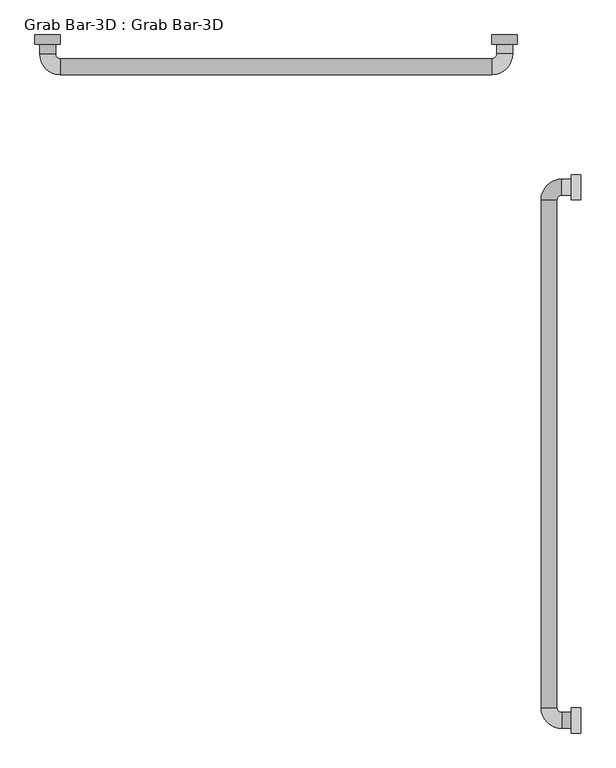
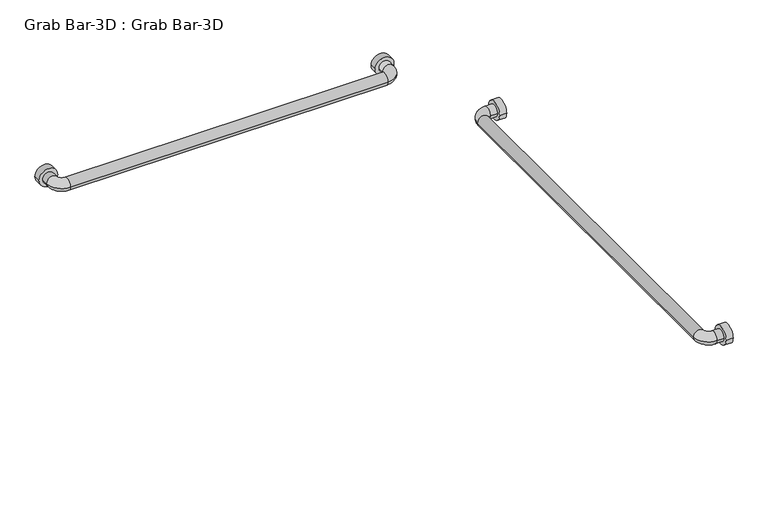
"""IFC4 building model written with IfcOpenShell, lengths in millimetres: proxy geometry, Grab Bar-3D : Grab Bar-3D."""

from ifc_helpers import new_model, si_unit, point, frame, frame_2d, origin, place, context, project, spatial, circle_curve, ellipse_curve, trimmed, segment, composite_curve, outline, extrude, source, transform, mapped, element, save
from ifc_brep_helpers import plane_surface, cylinder_surface, revolved_surface, advanced_brep


def grab_bar_3d_grab_bar_3d_a3ed3e83(model_context):
    return source(origin(), model_context, "Body", "SolidModel", [
        extrude(outline(composite_curve([segment(trimmed(circle_curve(frame_2d((-304.8, 914.4)), 25.4), [point((-279.4, 914.4))], [point((-330.2, 914.4))], False, "CARTESIAN"), True, "CONTINUOUS"), segment(trimmed(circle_curve(frame_2d((-304.8, 914.4)), 25.4), [point((-330.2, 914.4))], [point((-279.4, 914.4))], False, "CARTESIAN"), True, "CONTINUOUS")], self_intersect=False)), frame((-19.05, 0.0, 0.0), z_axis=(1.0, 0.0, 0.0), x_axis=(0.0, 1.0, 0.0)), (0.0, 0.0, 1.0), 19.05),
        extrude(outline(composite_curve([segment(trimmed(circle_curve(frame_2d((-1371.6, 914.4)), 25.4), [point((-1346.2, 914.4))], [point((-1397.0, 914.4))], False, "CARTESIAN"), True, "CONTINUOUS"), segment(trimmed(circle_curve(frame_2d((-1371.6, 914.4)), 25.4), [point((-1397.0, 914.4))], [point((-1346.2, 914.4))], False, "CARTESIAN"), True, "CONTINUOUS")], self_intersect=False)), frame((-19.05, 0.0, 0.0), z_axis=(1.0, 0.0, 0.0), x_axis=(0.0, 1.0, 0.0)), (0.0, 0.0, 1.0), 19.05),
        extrude(outline(composite_curve([segment(trimmed(circle_curve(frame_2d((914.4, -152.4)), 25.4), [point((914.4, -177.8))], [point((914.4, -127.0))], False, "CARTESIAN"), True, "CONTINUOUS"), segment(trimmed(circle_curve(frame_2d((914.4, -152.4)), 25.4), [point((914.4, -127.0))], [point((914.4, -177.8))], False, "CARTESIAN"), True, "CONTINUOUS")], self_intersect=False)), frame((0.0, -19.05, 0.0), z_axis=(0.0, 1.0, 0.0), x_axis=(0.0, 0.0, 1.0)), (0.0, 0.0, 1.0), 19.05),
        extrude(outline(composite_curve([segment(trimmed(circle_curve(frame_2d((914.4, -1066.8)), 25.4), [point((914.4, -1092.2))], [point((914.4, -1041.4))], False, "CARTESIAN"), True, "CONTINUOUS"), segment(trimmed(circle_curve(frame_2d((914.4, -1066.8)), 25.4), [point((914.4, -1041.4))], [point((914.4, -1092.2))], False, "CARTESIAN"), True, "CONTINUOUS")], self_intersect=False)), frame((0.0, -19.05, 0.0), z_axis=(0.0, 1.0, 0.0), x_axis=(0.0, 0.0, 1.0)), (0.0, 0.0, 1.0), 19.05),
        advanced_brep(
        [(-19.05, -320.675, 914.4), (-19.05, -288.925, 914.4), (-38.1, -288.925, 914.4), (-38.1, -320.675, 914.4), (-79.375, -330.2, 914.4), (-47.625, -330.2, 914.4), (-79.375, -1346.2, 914.4), (-47.625, -1346.2, 914.4), (-38.1, -1387.475, 914.4), (-38.1, -1355.725, 914.4), (-19.05, -1355.725, 914.4), (-19.05, -1387.475, 914.4)],
        [
            (0, 1, circle_curve(frame((-19.05, -304.8, 914.4), z_axis=(1.0, 0.0, 0.0), x_axis=(0.0, 1.0, 0.0)), 15.875)),
            (1, 0, circle_curve(frame((-19.05, -304.8, 914.4), z_axis=(1.0, 0.0, 0.0), x_axis=(0.0, 1.0, 0.0)), 15.875)),
            (1, 2),
            (2, 3, circle_curve(frame((-38.1, -304.8, 914.4), z_axis=(1.0, 0.0, 0.0), x_axis=(0.0, 1.0, 0.0)), 15.875)),
            (3, 0),
            (3, 2, circle_curve(frame((-38.1, -304.8, 914.4), z_axis=(1.0, 0.0, 0.0), x_axis=(0.0, 1.0, 0.0)), 15.875)),
            (4, 5, circle_curve(frame((-63.5, -330.2, 914.4), z_axis=(0.0, 1.0, 0.0), x_axis=(-1.0, 0.0, 0.0)), 15.875)),
            (5, 3, circle_curve(frame((-38.1, -330.2, 914.4), z_axis=(0.0, 0.0, -1.0), x_axis=(0.0, 1.0, 0.0)), 9.525)),
            (2, 4, circle_curve(frame((-38.1, -330.2, 914.4), z_axis=(0.0, 0.0, 1.0), x_axis=(0.0, 1.0, 0.0)), 41.275)),
            (5, 4, circle_curve(frame((-63.5, -330.2, 914.4), z_axis=(0.0, 1.0, 0.0), x_axis=(-1.0, 0.0, 0.0)), 15.875)),
            (4, 6),
            (6, 7, circle_curve(frame((-63.5, -1346.2, 914.4), z_axis=(0.0, 1.0, 0.0), x_axis=(-1.0, 0.0, 0.0)), 15.875)),
            (7, 5),
            (7, 6, circle_curve(frame((-63.5, -1346.2, 914.4), z_axis=(0.0, 1.0, 0.0), x_axis=(-1.0, 0.0, 0.0)), 15.875)),
            (8, 9, circle_curve(frame((-38.1, -1371.6, 914.4), z_axis=(-1.0, 0.0, 0.0), x_axis=(0.0, -1.0, 0.0)), 15.875)),
            (9, 7, circle_curve(frame((-38.1, -1346.2, 914.4), z_axis=(0.0, 0.0, -1.0), x_axis=(-1.0, 0.0, 0.0)), 9.525)),
            (6, 8, circle_curve(frame((-38.1, -1346.2, 914.4), z_axis=(0.0, 0.0, 1.0), x_axis=(-1.0, 0.0, 0.0)), 41.275)),
            (9, 8, circle_curve(frame((-38.1, -1371.6, 914.4), z_axis=(-1.0, 0.0, 0.0), x_axis=(0.0, -1.0, 0.0)), 15.875)),
            (10, 11, circle_curve(frame((-19.05, -1371.6, 914.4), z_axis=(1.0, 0.0, 0.0), x_axis=(0.0, -1.0, 0.0)), 15.875)),
            (11, 10, circle_curve(frame((-19.05, -1371.6, 914.4), z_axis=(1.0, 0.0, 0.0), x_axis=(0.0, -1.0, 0.0)), 15.875)),
            (8, 11),
            (10, 9),
        ],
        [
            plane_surface(frame((-19.05, -304.8, -930.275), z_axis=(1.0, 0.0, 0.0), x_axis=(0.0, 1.0, 0.0))),
            cylinder_surface(frame((-19.05, -304.8, 914.4), z_axis=(1.0, 0.0, 0.0), x_axis=(0.0, 1.0, 0.0)), 15.875),
            revolved_surface(trimmed(ellipse_curve(frame((-38.1, -304.8, 914.4), z_axis=(-1.0, 0.0, 0.0), x_axis=(0.0, 1.0, 0.0)), 15.875, 15.875), [point((-38.1, -320.675, 914.4))], [point((-38.1, -288.925, 914.4))], True, "CARTESIAN"), (-38.1, -330.2, 0.0), (0.0, 0.0, -1.0)),
            revolved_surface(trimmed(ellipse_curve(frame((-38.1, -304.8, 914.4), z_axis=(-1.0, 0.0, 0.0), x_axis=(0.0, 1.0, 0.0)), 15.875, 15.875), [point((-38.1, -288.925, 914.4))], [point((-38.1, -320.675, 914.4))], True, "CARTESIAN"), (-38.1, -330.2, 0.0), (0.0, 0.0, -1.0)),
            cylinder_surface(frame((-63.5, -330.2, 914.4), z_axis=(0.0, 1.0, 0.0), x_axis=(-1.0, 0.0, 0.0)), 15.875),
            revolved_surface(trimmed(ellipse_curve(frame((-63.5, -1346.2, 914.4), z_axis=(0.0, -1.0, 0.0), x_axis=(-1.0, 0.0, 0.0)), 15.875, 15.875), [point((-47.625, -1346.2, 914.4))], [point((-79.375, -1346.2, 914.4))], True, "CARTESIAN"), (-38.1, -1346.2, 0.0), (0.0, 0.0, -1.0)),
            revolved_surface(trimmed(ellipse_curve(frame((-63.5, -1346.2, 914.4), z_axis=(0.0, -1.0, 0.0), x_axis=(-1.0, 0.0, 0.0)), 15.875, 15.875), [point((-79.375, -1346.2, 914.4))], [point((-47.625, -1346.2, 914.4))], True, "CARTESIAN"), (-38.1, -1346.2, 0.0), (0.0, 0.0, -1.0)),
            plane_surface(frame((-19.05, -1371.6, -930.275), z_axis=(1.0, 0.0, 0.0), x_axis=(0.0, -1.0, 0.0))),
            cylinder_surface(frame((-38.1, -1371.6, 914.4), z_axis=(-1.0, 0.0, 0.0), x_axis=(0.0, -1.0, 0.0)), 15.875),
        ],
        [
            (0, [[1, 2]]),
            (1, [[3, 4, 5, -2]]),
            (1, [[-5, 6, -3, -1]]),
            (2, [[7, 8, -4, 9]]),
            (3, [[10, -9, -6, -8]]),
            (4, [[11, 12, 13, -7]]),
            (4, [[-13, 14, -11, -10]]),
            (5, [[15, 16, -12, 17]]),
            (6, [[18, -17, -14, -16]]),
            (7, [[19, 20]]),
            (8, [[21, -19, 22, -15]]),
            (8, [[-22, -20, -21, -18]]),
        ],
    ),
        advanced_brep(
        [(-1050.925, -19.05, 914.4), (-1082.675, -19.05, 914.4), (-1082.675, -38.1, 914.4), (-1050.925, -38.1, 914.4), (-1041.4, -79.375, 914.4), (-1041.4, -47.625, 914.4), (-177.8, -79.375, 914.4), (-177.8, -47.625, 914.4), (-136.525, -38.1, 914.4), (-168.275, -38.1, 914.4), (-168.275, -19.05, 914.4), (-136.525, -19.05, 914.4)],
        [
            (0, 1, circle_curve(frame((-1066.8, -19.05, 914.4), z_axis=(0.0, 1.0, 0.0), x_axis=(-1.0, 0.0, 0.0)), 15.875)),
            (1, 0, circle_curve(frame((-1066.8, -19.05, 914.4), z_axis=(0.0, 1.0, 0.0), x_axis=(-1.0, 0.0, 0.0)), 15.875)),
            (1, 2),
            (2, 3, circle_curve(frame((-1066.8, -38.1, 914.4), z_axis=(0.0, 1.0, 0.0), x_axis=(-1.0, 0.0, 0.0)), 15.875)),
            (3, 0),
            (3, 2, circle_curve(frame((-1066.8, -38.1, 914.4), z_axis=(0.0, 1.0, 0.0), x_axis=(-1.0, 0.0, 0.0)), 15.875)),
            (4, 5, circle_curve(frame((-1041.4, -63.5, 914.4), z_axis=(-1.0, 0.0, 0.0), x_axis=(0.0, -1.0, 0.0)), 15.875)),
            (5, 3, circle_curve(frame((-1041.4, -38.1, 914.4), z_axis=(0.0, 0.0, -1.0), x_axis=(-1.0, 0.0, 0.0)), 9.525)),
            (2, 4, circle_curve(frame((-1041.4, -38.1, 914.4), z_axis=(0.0, 0.0, 1.0), x_axis=(-1.0, 0.0, 0.0)), 41.275)),
            (5, 4, circle_curve(frame((-1041.4, -63.5, 914.4), z_axis=(-1.0, 0.0, 0.0), x_axis=(0.0, -1.0, 0.0)), 15.875)),
            (4, 6),
            (6, 7, circle_curve(frame((-177.8, -63.5, 914.4), z_axis=(-1.0, 0.0, 0.0), x_axis=(0.0, -1.0, 0.0)), 15.875)),
            (7, 5),
            (7, 6, circle_curve(frame((-177.8, -63.5, 914.4), z_axis=(-1.0, 0.0, 0.0), x_axis=(0.0, -1.0, 0.0)), 15.875)),
            (8, 9, circle_curve(frame((-152.4, -38.1, 914.4), z_axis=(0.0, -1.0, 0.0), x_axis=(1.0, 0.0, 0.0)), 15.875)),
            (9, 7, circle_curve(frame((-177.8, -38.1, 914.4), z_axis=(0.0, 0.0, -1.0), x_axis=(0.0, -1.0, 0.0)), 9.525)),
            (6, 8, circle_curve(frame((-177.8, -38.1, 914.4), z_axis=(0.0, 0.0, 1.0), x_axis=(0.0, -1.0, 0.0)), 41.275)),
            (9, 8, circle_curve(frame((-152.4, -38.1, 914.4), z_axis=(0.0, -1.0, 0.0), x_axis=(1.0, 0.0, 0.0)), 15.875)),
            (10, 11, circle_curve(frame((-152.4, -19.05, 914.4), z_axis=(0.0, 1.0, 0.0), x_axis=(1.0, 0.0, 0.0)), 15.875)),
            (11, 10, circle_curve(frame((-152.4, -19.05, 914.4), z_axis=(0.0, 1.0, 0.0), x_axis=(1.0, 0.0, 0.0)), 15.875)),
            (8, 11),
            (10, 9),
        ],
        [
            plane_surface(frame((-1997.075, -19.05, 0.0), z_axis=(0.0, 1.0, 0.0), x_axis=(0.0, 0.0, 1.0))),
            cylinder_surface(frame((-1066.8, -19.05, 914.4), z_axis=(0.0, 1.0, 0.0), x_axis=(-1.0, 0.0, 0.0)), 15.875),
            revolved_surface(trimmed(ellipse_curve(frame((-1066.8, -38.1, 914.4), z_axis=(0.0, -1.0, 0.0), x_axis=(-1.0, 0.0, 0.0)), 15.875, 15.875), [point((-1050.925, -38.1, 914.4))], [point((-1082.675, -38.1, 914.4))], True, "CARTESIAN"), (-1041.4, -38.1, 0.0), (0.0, 0.0, -1.0)),
            revolved_surface(trimmed(ellipse_curve(frame((-1066.8, -38.1, 914.4), z_axis=(0.0, -1.0, 0.0), x_axis=(-1.0, 0.0, 0.0)), 15.875, 15.875), [point((-1082.675, -38.1, 914.4))], [point((-1050.925, -38.1, 914.4))], True, "CARTESIAN"), (-1041.4, -38.1, 0.0), (0.0, 0.0, -1.0)),
            cylinder_surface(frame((-1041.4, -63.5, 914.4), z_axis=(-1.0, 0.0, 0.0), x_axis=(0.0, -1.0, 0.0)), 15.875),
            revolved_surface(trimmed(ellipse_curve(frame((-177.8, -63.5, 914.4), z_axis=(1.0, 0.0, 0.0), x_axis=(0.0, -1.0, 0.0)), 15.875, 15.875), [point((-177.8, -47.625, 914.4))], [point((-177.8, -79.375, 914.4))], True, "CARTESIAN"), (-177.8, -38.1, 0.0), (0.0, 0.0, -1.0)),
            revolved_surface(trimmed(ellipse_curve(frame((-177.8, -63.5, 914.4), z_axis=(1.0, 0.0, 0.0), x_axis=(0.0, -1.0, 0.0)), 15.875, 15.875), [point((-177.8, -79.375, 914.4))], [point((-177.8, -47.625, 914.4))], True, "CARTESIAN"), (-177.8, -38.1, 0.0), (0.0, 0.0, -1.0)),
            plane_surface(frame((-1082.675, -19.05, 0.0), z_axis=(0.0, 1.0, 0.0), x_axis=(0.0, 0.0, -1.0))),
            cylinder_surface(frame((-152.4, -38.1, 914.4), z_axis=(0.0, -1.0, 0.0), x_axis=(1.0, 0.0, 0.0)), 15.875),
        ],
        [
            (0, [[1, 2]]),
            (1, [[3, 4, 5, -2]]),
            (1, [[-5, 6, -3, -1]]),
            (2, [[7, 8, -4, 9]]),
            (3, [[10, -9, -6, -8]]),
            (4, [[11, 12, 13, -7]]),
            (4, [[-13, 14, -11, -10]]),
            (5, [[15, 16, -12, 17]]),
            (6, [[18, -17, -14, -16]]),
            (7, [[19, 20]]),
            (8, [[21, -19, 22, -15]]),
            (8, [[-22, -20, -21, -18]]),
        ],
    ),
    ])


if __name__ == "__main__":
    model = new_model("IFC4")
    model_context = context("Model", 3, world=origin())
    ifc_project = project(units=[si_unit("LENGTHUNIT", "METRE", prefix="MILLI")], contexts=[model_context])
    site = spatial("IfcSite", under=ifc_project)
    building = spatial("IfcBuilding", under=site)
    placement = place(None, origin())
    grab_bar_3d_grab_bar_3d_shape = grab_bar_3d_grab_bar_3d_a3ed3e83(model_context)
    element("IfcBuildingElementProxy", 1, Name="Grab Bar-3D : Grab Bar-3D", ObjectType="Grab Bar-3D : Grab Bar-3D", at=placement, inside=building, context=model_context, shape_type="MappedRepresentation", body=[
        mapped(grab_bar_3d_grab_bar_3d_shape, transform((0.0, 0.0, 0.0), x_axis=(1.0, 0.0, 0.0), y_axis=(0.0, 1.0, 0.0), z_axis=(0.0, 0.0, 1.0))),
    ])
    save(model, "model.ifc")

# Revit data of these elements
# Type "Grab Bar-3D : Grab Bar-3D"
#   Assembly Code = "C1030200"
#   Back Bar Length = 3' - 0"
#   Mounting Height = 3' - 0"
#   Side Bar Length = 3' - 6"
#   Default Elevation = 0
# Element 1 (IfcBuildingElementProxy, "Grab Bar-3D : Grab Bar-3D")
#   Materials on its faces: "Metal - Aluminum, Brushed"
# Materials
#   "Metal - Aluminum, Brushed": class "Unassigned", colour RGB 247 247 247, transparency 0
